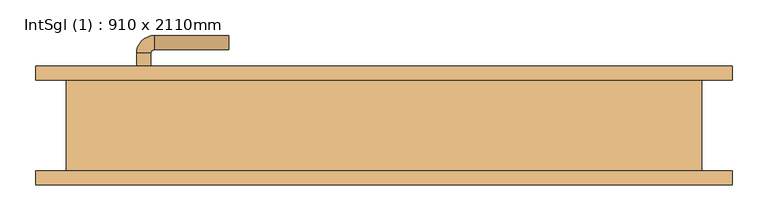
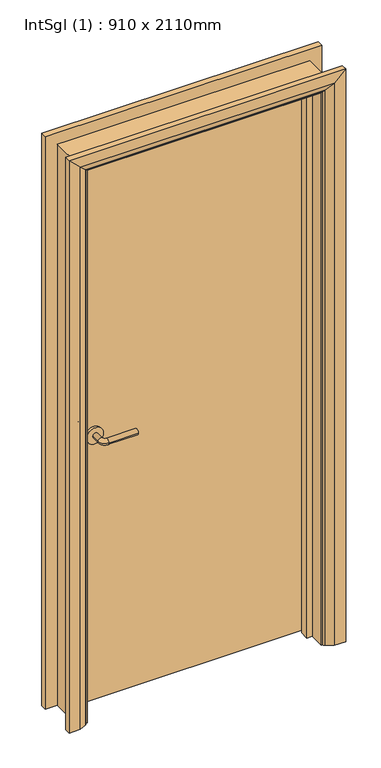
"""IFC4 building model written with IfcOpenShell, lengths in millimetres: door geometry, IntSgl (1) : 910 x 2110mm."""

from ifc_helpers import new_model, si_unit, point, frame, frame_2d, origin, place, context, project, spatial, polyline, circle_curve, ellipse_curve, trimmed, segment, composite_curve, outline, extrude, faceted_brep, source, transform, mapped, element, save
from ifc_brep_helpers import plane_surface, cylinder_surface, revolved_surface, advanced_brep


def intsgl_1_910_x_2110mm_8bdb4243(model_context):
    return source(origin(), model_context, "Body", "SolidModel", [
        advanced_brep(
        [(-348.0, 17.75, 1000.0), (-328.0, 17.75, 1000.0), (-328.0, -12.25, 1000.0), (-348.0, -12.25, 1000.0), (-323.0, -17.25, 1000.0), (-323.0, -37.25, 1000.0), (-218.0, -37.25, 1000.0), (-218.0, -17.25, 1000.0)],
        [
            (0, 1, circle_curve(frame((-338.0, 17.75, 1000.0), z_axis=(0.0, 1.0, 0.0), x_axis=(1.0, 0.0, 0.0)), 10.0)),
            (1, 0, circle_curve(frame((-338.0, 17.75, 1000.0), z_axis=(0.0, 1.0, 0.0), x_axis=(1.0, 0.0, 0.0)), 10.0)),
            (1, 2),
            (2, 3, circle_curve(frame((-338.0, -12.25, 1000.0), z_axis=(0.0, 1.0, 0.0), x_axis=(1.0, 0.0, 0.0)), 10.0)),
            (3, 0),
            (3, 2, circle_curve(frame((-338.0, -12.25, 1000.0), z_axis=(0.0, 1.0, 0.0), x_axis=(1.0, 0.0, 0.0)), 10.0)),
            (4, 5, circle_curve(frame((-323.0, -27.25, 1000.0), z_axis=(-1.0, 0.0, 0.0), x_axis=(0.0, 1.0, 0.0)), 10.0)),
            (5, 3, circle_curve(frame((-323.0, -12.25, 1000.0), z_axis=(0.0, 0.0, -1.0), x_axis=(-1.0, 0.0, 0.0)), 25.0)),
            (2, 4, circle_curve(frame((-323.0, -12.25, 1000.0), z_axis=(0.0, 0.0, 1.0), x_axis=(-1.0, 0.0, 0.0)), 5.0)),
            (5, 4, circle_curve(frame((-323.0, -27.25, 1000.0), z_axis=(-1.0, 0.0, 0.0), x_axis=(0.0, 1.0, 0.0)), 10.0)),
            (6, 7, circle_curve(frame((-218.0, -27.25, 1000.0), z_axis=(1.0, 0.0, 0.0), x_axis=(0.0, 1.0, 0.0)), 10.0)),
            (7, 6, circle_curve(frame((-218.0, -27.25, 1000.0), z_axis=(1.0, 0.0, 0.0), x_axis=(0.0, 1.0, 0.0)), 10.0)),
            (4, 7),
            (6, 5),
        ],
        [
            plane_surface(frame((-338.0, 17.75, 1000.0), z_axis=(0.0, 1.0, 0.0), x_axis=(0.0, 0.0, 1.0))),
            cylinder_surface(frame((-338.0, 17.75, 1000.0), z_axis=(0.0, 1.0, 0.0), x_axis=(1.0, 0.0, 0.0)), 10.0),
            revolved_surface(trimmed(ellipse_curve(frame((-338.0, -12.25, 1000.0), z_axis=(0.0, -1.0, 0.0), x_axis=(1.0, 0.0, 0.0)), 10.0, 10.0), [point((-348.0, -12.25, 1000.0))], [point((-328.0, -12.25, 1000.0))], True, "CARTESIAN"), (-323.0, -12.25, 1000.0), (0.0, 0.0, -1.0)),
            revolved_surface(trimmed(ellipse_curve(frame((-338.0, -12.25, 1000.0), z_axis=(0.0, -1.0, 0.0), x_axis=(1.0, 0.0, 0.0)), 10.0, 10.0), [point((-328.0, -12.25, 1000.0))], [point((-348.0, -12.25, 1000.0))], True, "CARTESIAN"), (-323.0, -12.25, 1000.0), (0.0, 0.0, -1.0)),
            plane_surface(frame((-218.0, -27.25, 1000.0), z_axis=(1.0, 0.0, 0.0), x_axis=(0.0, 0.0, 1.0))),
            cylinder_surface(frame((-323.0, -27.25, 1000.0), z_axis=(-1.0, 0.0, 0.0), x_axis=(0.0, 1.0, 0.0)), 10.0),
        ],
        [
            (0, [[1, 2]]),
            (1, [[3, 4, 5, -2]]),
            (1, [[-5, 6, -3, -1]]),
            (2, [[7, 8, -4, 9]]),
            (3, [[10, -9, -6, -8]]),
            (4, [[11, 12]]),
            (5, [[13, -11, 14, -7]]),
            (5, [[-14, -12, -13, -10]]),
        ],
    ),
        extrude(outline(composite_curve([segment(trimmed(circle_curve(frame_2d((1000.0, -340.5)), 30.0), [point((1000.0, -370.5))], [point((1000.0, -310.5))], False, "CARTESIAN"), True, "CONTINUOUS"), segment(trimmed(circle_curve(frame_2d((1000.0, -340.5)), 30.0), [point((1000.0, -310.5))], [point((1000.0, -370.5))], False, "CARTESIAN"), True, "CONTINUOUS")], self_intersect=False)), frame((0.0, 17.75, 0.0), z_axis=(0.0, 1.0, 0.0), x_axis=(0.0, 0.0, 1.0)), (0.0, 0.0, 1.0), 8.0),
        advanced_brep(
        [(-348.0, 71.75, 1000.0), (-328.0, 71.75, 1000.0), (-348.0, 101.75, 1000.0), (-328.0, 101.75, 1000.0), (-323.0, 106.75, 1000.0), (-323.0, 126.75, 1000.0), (-218.0, 126.75, 1000.0), (-218.0, 106.75, 1000.0)],
        [
            (0, 1, circle_curve(frame((-338.0, 71.75, 1000.0), z_axis=(0.0, -1.0, 0.0), x_axis=(1.0, 0.0, 0.0)), 10.0)),
            (1, 0, circle_curve(frame((-338.0, 71.75, 1000.0), z_axis=(0.0, -1.0, 0.0), x_axis=(1.0, 0.0, 0.0)), 10.0)),
            (0, 2),
            (2, 3, circle_curve(frame((-338.0, 101.75, 1000.0), z_axis=(0.0, -1.0, 0.0), x_axis=(1.0, 0.0, 0.0)), 10.0)),
            (3, 1),
            (3, 2, circle_curve(frame((-338.0, 101.75, 1000.0), z_axis=(0.0, -1.0, 0.0), x_axis=(1.0, 0.0, 0.0)), 10.0)),
            (4, 3, circle_curve(frame((-323.0, 101.75, 1000.0), z_axis=(0.0, 0.0, 1.0), x_axis=(-1.0, 0.0, 0.0)), 5.0)),
            (2, 5, circle_curve(frame((-323.0, 101.75, 1000.0), z_axis=(0.0, 0.0, -1.0), x_axis=(-1.0, 0.0, 0.0)), 25.0)),
            (5, 4, circle_curve(frame((-323.0, 116.75, 1000.0), z_axis=(-1.0, 0.0, 0.0), x_axis=(0.0, -1.0, 0.0)), 10.0)),
            (4, 5, circle_curve(frame((-323.0, 116.75, 1000.0), z_axis=(-1.0, 0.0, 0.0), x_axis=(0.0, -1.0, 0.0)), 10.0)),
            (6, 7, circle_curve(frame((-218.0, 116.75, 1000.0), z_axis=(1.0, 0.0, 0.0), x_axis=(0.0, -1.0, 0.0)), 10.0)),
            (7, 6, circle_curve(frame((-218.0, 116.75, 1000.0), z_axis=(1.0, 0.0, 0.0), x_axis=(0.0, -1.0, 0.0)), 10.0)),
            (5, 6),
            (7, 4),
        ],
        [
            plane_surface(frame((-338.0, 71.75, 1000.0), z_axis=(0.0, -1.0, 0.0), x_axis=(0.0, 0.0, 1.0))),
            cylinder_surface(frame((-338.0, 71.75, 1000.0), z_axis=(0.0, -1.0, 0.0), x_axis=(1.0, 0.0, 0.0)), 10.0),
            revolved_surface(trimmed(ellipse_curve(frame((-338.0, 101.75, 1000.0), z_axis=(0.0, -1.0, 0.0), x_axis=(1.0, 0.0, 0.0)), 10.0, 10.0), [point((-348.0, 101.75, 1000.0))], [point((-328.0, 101.75, 1000.0))], True, "CARTESIAN"), (-323.0, 101.75, 1000.0), (0.0, 0.0, -1.0)),
            revolved_surface(trimmed(ellipse_curve(frame((-338.0, 101.75, 1000.0), z_axis=(0.0, -1.0, 0.0), x_axis=(1.0, 0.0, 0.0)), 10.0, 10.0), [point((-328.0, 101.75, 1000.0))], [point((-348.0, 101.75, 1000.0))], True, "CARTESIAN"), (-323.0, 101.75, 1000.0), (0.0, 0.0, -1.0)),
            plane_surface(frame((-218.0, 116.75, 1000.0), z_axis=(1.0, 0.0, 0.0), x_axis=(0.0, 0.0, 1.0))),
            cylinder_surface(frame((-323.0, 116.75, 1000.0), z_axis=(-1.0, 0.0, 0.0), x_axis=(0.0, -1.0, 0.0)), 10.0),
        ],
        [
            (0, [[1, 2]]),
            (1, [[-1, 3, 4, 5]]),
            (1, [[-2, -5, 6, -3]]),
            (2, [[7, -4, 8, 9]]),
            (3, [[-8, -6, -7, 10]]),
            (4, [[11, 12]]),
            (5, [[-9, 13, -12, 14]]),
            (5, [[-10, -14, -11, -13]]),
        ],
    ),
        extrude(outline(composite_curve([segment(trimmed(circle_curve(frame_2d((1000.0, -340.5)), 30.0), [point((1000.0, -370.5))], [point((1000.0, -310.5))], False, "CARTESIAN"), True, "CONTINUOUS"), segment(trimmed(circle_curve(frame_2d((1000.0, -340.5)), 30.0), [point((1000.0, -310.5))], [point((1000.0, -370.5))], False, "CARTESIAN"), True, "CONTINUOUS")], self_intersect=False)), frame((0.0, 63.75, 0.0), z_axis=(0.0, 1.0, 0.0), x_axis=(0.0, 0.0, 1.0)), (0.0, 0.0, 1.0), 8.0),
        extrude(outline(polyline([(413.0, 25.75), (-413.0, 25.75), (-413.0, 63.75), (413.0, 63.75), (413.0, 25.75)])), frame((0.0, 0.0, 8.0), z_axis=(0.0, 0.0, 1.0), x_axis=(1.0, 0.0, 0.0)), (0.0, 0.0, 1.0), 2060.0),
        advanced_brep(
        [(490.0, 83.75, 0.0), (490.0, 63.75, 0.0), (420.0, 63.75, 0.0), (424.0, 69.75, 0.0), (450.0, 83.75, 0.0), (490.0, 83.75, 2145.0), (490.0, 63.75, 2145.0), (-490.0, 63.75, 2145.0), (-490.0, 63.75, 0.0), (-420.0, 63.75, 0.0), (-420.0, 63.75, 2075.0), (420.0, 63.75, 2075.0), (424.0, 69.75, 2079.0), (450.0, 83.75, 2105.0), (-450.0, 83.75, 2105.0), (-450.0, 83.75, 0.0), (-490.0, 83.75, 0.0), (-490.0, 83.75, 2145.0), (-424.0, 69.75, 2079.0), (-424.0, 69.75, 0.0)],
        [
            (0, 1),
            (1, 2),
            (2, 3, circle_curve(frame((428.0, 62.75, 0.0), z_axis=(0.0, 0.0, -1.0), x_axis=(1.0, 0.0, 0.0)), 8.0622577)),
            (3, 4),
            (4, 0),
            (0, 5),
            (5, 6),
            (6, 1),
            (6, 7),
            (7, 8),
            (8, 9),
            (9, 10),
            (10, 11),
            (11, 2),
            (11, 12, ellipse_curve(frame((428.0, 62.75, 2083.0), z_axis=(0.7071067811865475, 0.0, -0.7071067811865475), x_axis=(-0.7071067811865474, 0.0, -0.7071067811865476)), 11.4017543, 8.0622577)),
            (12, 3),
            (12, 13),
            (13, 4),
            (13, 14),
            (14, 15),
            (15, 16),
            (16, 17),
            (17, 5),
            (17, 7),
            (10, 18, ellipse_curve(frame((-428.0, 62.75, 2083.0), z_axis=(0.7071067811865475, 0.0, 0.7071067811865475), x_axis=(0.7071067811865476, 0.0, -0.7071067811865474)), 11.4017543, 8.0622577)),
            (18, 12),
            (18, 14),
            (15, 19),
            (19, 9, circle_curve(frame((-428.0, 62.75, 0.0), z_axis=(0.0, 0.0, -1.0), x_axis=(-1.0, 0.0, 0.0)), 8.0622577)),
            (8, 16),
            (19, 18),
        ],
        [
            plane_surface(frame((420.0, 63.75, 0.0), z_axis=(0.0, 0.0, -1.0), x_axis=(0.0, -1.0, 0.0))),
            plane_surface(frame((490.0, 83.75, 0.0), z_axis=(1.0, 0.0, 0.0), x_axis=(0.0, 0.0, 1.0))),
            plane_surface(frame((490.0, 63.75, 0.0), z_axis=(0.0, -1.0, 0.0), x_axis=(0.0, 0.0, 1.0))),
            cylinder_surface(frame((428.0, 62.75, 0.0), z_axis=(0.0, 0.0, -1.0), x_axis=(1.0, 0.0, 0.0)), 8.0622577),
            plane_surface(frame((424.0, 69.75, 0.0), z_axis=(-0.4740998230350126, 0.880471099922178, 0.0), x_axis=(0.0, 0.0, 1.0))),
            plane_surface(frame((450.0, 83.75, 0.0), z_axis=(0.0, 1.0, 0.0), x_axis=(0.0, 0.0, 1.0))),
            plane_surface(frame((490.0, 83.75, 2145.0), z_axis=(0.0, 0.0, 1.0), x_axis=(-1.0, 0.0, 0.0))),
            cylinder_surface(frame((420.0, 62.75, 2083.0), z_axis=(1.0, 0.0, 0.0), x_axis=(0.0, 0.0, 1.0)), 8.0622577),
            plane_surface(frame((424.0, 69.75, 2079.0), z_axis=(0.0, 0.8804710999221764, -0.4740998230350154), x_axis=(-1.0, 0.0, 0.0))),
            plane_surface(frame((-420.0, 63.75, 0.0), z_axis=(0.0, 0.0, -1.0), x_axis=(0.0, -1.0, 0.0))),
            plane_surface(frame((-490.0, 83.75, 2145.0), z_axis=(-1.0, 0.0, 0.0), x_axis=(0.0, 0.0, -1.0))),
            cylinder_surface(frame((-428.0, 62.75, 2075.0), z_axis=(0.0, 0.0, 1.0), x_axis=(-1.0, 0.0, 0.0)), 8.0622577),
            plane_surface(frame((-424.0, 69.75, 2079.0), z_axis=(0.47409982303501824, 0.8804710999221749, 0.0), x_axis=(0.0, 0.0, -1.0))),
        ],
        [
            (0, [[1, 2, 3, 4, 5]]),
            (1, [[-1, 6, 7, 8]]),
            (2, [[-2, -8, 9, 10, 11, 12, 13, 14]]),
            (3, [[-3, -14, 15, 16]]),
            (4, [[-4, -16, 17, 18]]),
            (5, [[-5, -18, 19, 20, 21, 22, 23, -6]]),
            (6, [[-7, -23, 24, -9]]),
            (7, [[-15, -13, 25, 26]]),
            (8, [[-17, -26, 27, -19]]),
            (9, [[-21, 28, 29, -11, 30]]),
            (10, [[-24, -22, -30, -10]]),
            (11, [[-25, -12, -29, 31]]),
            (12, [[-27, -31, -28, -20]]),
        ],
    ),
        extrude(outline(polyline([(0.0, -415.0), (0.0, -396.0), (2051.0, -396.0), (2051.0, 396.0), (0.0, 396.0), (0.0, 415.0), (2070.0, 415.0), (2070.0, -415.0), (0.0, -415.0)])), frame((0.0, -8.25, 0.0), z_axis=(0.0, 1.0, 0.0), x_axis=(0.0, 0.0, 1.0)), (0.0, 0.0, 1.0), 32.0),
        advanced_brep(
        [(-490.0, -83.75, 0.0), (-490.0, -63.75, 0.0), (-420.0, -63.75, 0.0), (-424.0, -69.75, 0.0), (-450.0, -83.75, 0.0), (-490.0, -83.75, 2145.0), (-490.0, -63.75, 2145.0), (-420.0, -63.75, 2075.0), (-424.0, -69.75, 2079.0), (-450.0, -83.75, 2105.0), (490.0, -83.75, 2145.0), (490.0, -63.75, 2145.0), (420.0, -63.75, 2075.0), (424.0, -69.75, 2079.0), (450.0, -83.75, 2105.0), (490.0, -83.75, 0.0), (450.0, -83.75, 0.0), (424.0, -69.75, 0.0), (420.0, -63.75, 0.0), (490.0, -63.75, 0.0)],
        [
            (0, 1),
            (1, 2),
            (2, 3, circle_curve(frame((-428.0, -62.75, 0.0), z_axis=(0.0, 0.0, -1.0), x_axis=(-1.0, 0.0, 0.0)), 8.0622577)),
            (3, 4),
            (4, 0),
            (0, 5),
            (5, 6),
            (6, 1),
            (6, 7),
            (7, 2),
            (7, 8, ellipse_curve(frame((-428.0, -62.75, 2083.0), z_axis=(-0.7071067811865475, 0.0, -0.7071067811865475), x_axis=(0.7071067811865474, 0.0, -0.7071067811865476)), 11.4017543, 8.0622577)),
            (8, 3),
            (8, 9),
            (9, 4),
            (9, 5),
            (5, 10),
            (10, 11),
            (11, 6),
            (11, 12),
            (12, 7),
            (12, 13, ellipse_curve(frame((428.0, -62.75, 2083.0), z_axis=(-0.7071067811865475, 0.0, 0.7071067811865475), x_axis=(-0.7071067811865476, 0.0, -0.7071067811865474)), 11.4017543, 8.0622577)),
            (13, 8),
            (13, 14),
            (14, 9),
            (14, 10),
            (15, 16),
            (16, 17),
            (17, 18, circle_curve(frame((428.0, -62.75, 0.0), z_axis=(0.0, 0.0, -1.0), x_axis=(1.0, 0.0, 0.0)), 8.0622577)),
            (18, 19),
            (19, 15),
            (10, 15),
            (19, 11),
            (18, 12),
            (17, 13),
            (16, 14),
        ],
        [
            plane_surface(frame((-420.0, -136.5510989, 0.0), z_axis=(0.0, 0.0, -1.0), x_axis=(1.0, 0.0, 0.0))),
            plane_surface(frame((-490.0, -83.75, 0.0), z_axis=(-1.0, 0.0, 0.0), x_axis=(0.0, 0.0, 1.0))),
            plane_surface(frame((-490.0, -63.75, 0.0), z_axis=(0.0, 1.0, 0.0), x_axis=(0.0, 0.0, 1.0))),
            cylinder_surface(frame((-428.0, -62.75, 0.0), z_axis=(0.0, 0.0, -1.0), x_axis=(-1.0, 0.0, 0.0)), 8.0622577),
            plane_surface(frame((-424.0, -69.75, 0.0), z_axis=(0.4740998230350183, -0.8804710999221749, 0.0), x_axis=(0.0, 0.0, 1.0))),
            plane_surface(frame((-450.0, -83.75, 0.0), z_axis=(0.0, -1.0, 0.0), x_axis=(0.0, 0.0, 1.0))),
            plane_surface(frame((-490.0, -83.75, 2145.0), z_axis=(0.0, 0.0, 1.0), x_axis=(1.0, 0.0, 0.0))),
            plane_surface(frame((-490.0, -63.75, 2145.0), z_axis=(0.0, 1.0, 0.0), x_axis=(1.0, 0.0, 0.0))),
            cylinder_surface(frame((-420.0, -62.75, 2083.0), z_axis=(-1.0, 0.0, 0.0), x_axis=(0.0, 0.0, 1.0)), 8.0622577),
            plane_surface(frame((-424.0, -69.75, 2079.0), z_axis=(0.0, -0.8804710999221749, -0.4740998230350183), x_axis=(1.0, 0.0, 0.0))),
            plane_surface(frame((-450.0, -83.75, 2105.0), z_axis=(0.0, -1.0, 0.0), x_axis=(1.0, 0.0, 0.0))),
            plane_surface(frame((420.0, -136.5510989, 0.0), z_axis=(0.0, 0.0, -1.0), x_axis=(-1.0, 0.0, 0.0))),
            plane_surface(frame((490.0, -83.75, 2145.0), z_axis=(1.0, 0.0, 0.0), x_axis=(0.0, 0.0, -1.0))),
            plane_surface(frame((490.0, -63.75, 2145.0), z_axis=(0.0, 1.0, 0.0), x_axis=(0.0, 0.0, -1.0))),
            cylinder_surface(frame((428.0, -62.75, 2075.0), z_axis=(0.0, 0.0, 1.0), x_axis=(1.0, 0.0, 0.0)), 8.0622577),
            plane_surface(frame((424.0, -69.75, 2079.0), z_axis=(-0.4740998230350183, -0.8804710999221749, 0.0), x_axis=(0.0, 0.0, -1.0))),
            plane_surface(frame((450.0, -83.75, 2105.0), z_axis=(0.0, -1.0, 0.0), x_axis=(0.0, 0.0, -1.0))),
        ],
        [
            (0, [[1, 2, 3, 4, 5]]),
            (1, [[-1, 6, 7, 8]]),
            (2, [[-2, -8, 9, 10]]),
            (3, [[-3, -10, 11, 12]]),
            (4, [[-4, -12, 13, 14]]),
            (5, [[-5, -14, 15, -6]]),
            (6, [[-7, 16, 17, 18]]),
            (7, [[-9, -18, 19, 20]]),
            (8, [[-11, -20, 21, 22]]),
            (9, [[-13, -22, 23, 24]]),
            (10, [[-15, -24, 25, -16]]),
            (11, [[26, 27, 28, 29, 30]]),
            (12, [[-17, 31, -30, 32]]),
            (13, [[-19, -32, -29, 33]]),
            (14, [[-21, -33, -28, 34]]),
            (15, [[-23, -34, -27, 35]]),
            (16, [[-25, -35, -26, -31]]),
        ],
    ),
        faceted_brep([(-415.0, 63.75, 0.0), (-415.0, -63.75, 0.0), (-447.0, -63.75, 0.0), (-447.0, 63.75, 0.0), (-415.0, 63.75, 2070.0), (-415.0, -63.75, 2070.0), (-447.0, -63.75, 2102.0), (-447.0, 63.75, 2102.0), (415.0, 63.75, 2070.0), (415.0, -63.75, 2070.0), (447.0, -63.75, 2102.0), (447.0, 63.75, 2102.0), (415.0, 63.75, 0.0), (447.0, 63.75, 0.0), (447.0, -63.75, 0.0), (415.0, -63.75, 0.0)], [[[0, 1, 2, 3]], [[1, 0, 4, 5]], [[2, 1, 5, 6]], [[3, 2, 6, 7]], [[0, 3, 7, 4]], [[5, 4, 8, 9]], [[6, 5, 9, 10]], [[7, 6, 10, 11]], [[4, 7, 11, 8]], [[12, 13, 14, 15]], [[9, 8, 12, 15]], [[10, 9, 15, 14]], [[11, 10, 14, 13]], [[8, 11, 13, 12]]]),
    ])


if __name__ == "__main__":
    model = new_model("IFC4")
    model_context = context("Model", 3, world=origin())
    ifc_project = project(units=[si_unit("LENGTHUNIT", "METRE", prefix="MILLI")], contexts=[model_context])
    site = spatial("IfcSite", under=ifc_project)
    building = spatial("IfcBuilding", under=site)
    placement = place(None, origin())
    intsgl_1_910_x_2110mm_shape = intsgl_1_910_x_2110mm_8bdb4243(model_context)
    element("IfcDoor", 1, ObjectType="IntSgl (1) : 910 x 2110mm", at=placement, inside=building, context=model_context, shape_type="MappedRepresentation", body=[
        mapped(intsgl_1_910_x_2110mm_shape, transform((0.0, 0.0, 0.0), x_axis=(1.0, 0.0, 0.0), y_axis=(0.0, 1.0, 0.0), z_axis=(0.0, 0.0, 1.0))),
    ])
    save(model, "model.ifc")

# Revit data of these elements
# Type "IntSgl (1) : 910 x 2110mm"
#   Construction Type Id = "MDOOR"
#   Analytic Construction = "Metal"
#   Type Mark = "41"
#   Type Comments = "Internal Single"
#   Operation = "SingleSwingRight"
#   Manufacturer = "Revit"
#   Keynote = "L20"
#   Description = "Internal Single Door"
#   Visual Light Transmittance = 0
#   Solar Heat Gain Coefficient = 0
#   Heat Transfer Coefficient (U) = 3.7021 W/(m²·K)
#   UnderCut = 8 mm
#   Tolerance = 2 mm
#   Thickness = 38 mm
#   Structural Tolerance = 8 mm
#   StopDepth = 32 mm
#   Stop Thickness = 19 mm
#   Rough Width = 910 mm
#   Rough Height = 2110 mm
#   Height to Top Lock Rail = 1000 mm
#   Handle Z Distance = 1000 mm
#   Handle X Distance = 75 mm
#   Frame Thickness = 32 mm
#   Door Panel Width = 826 mm
#   Door Panel Thickness = 38 mm
#   Door Panel Offset = 0 mm
#   Height = 2110 mm
#   Width = 910 mm
#   Door Panel Height = 2060 mm
#   Architrave Setback = 5 mm
#   Function = 0
#   Vis - Ironmongery = yes
#   Material Ironmongery = Door - Handle
#   Material Frame = Door - Frame/Mullion (1)
#   Material Door = Door - Panel
#   Material Architrave = Door - Architrave
#   Wall Closure = (empty or 0)
# Element 1 (IfcDoor, "IntSgl (1) : 910 x 2110mm")
#   Materials on its faces: "Door - Architrave", "Door - Handle", "Door - Frame/Mullion (1)", "Door - Panel"
# Materials
#   "Door - Handle": class "Miscellaneous", colour RGB 0 0 0, transparency 0, Keynote = "P21"
#   "Door - Frame/Mullion (1)": class "Wood", colour RGB 212 179 113, transparency 0, Keynote = "L20", Cost = 0
#   "Door - Panel": class "Wood", colour RGB 210 159 95, transparency 0, Keynote = "L20"
#   "Door - Architrave": class "Wood", colour RGB 154 90 5, transparency 0, Keynote = "P20"
